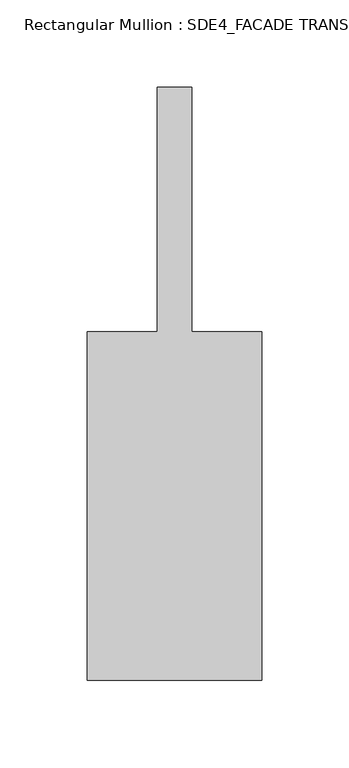
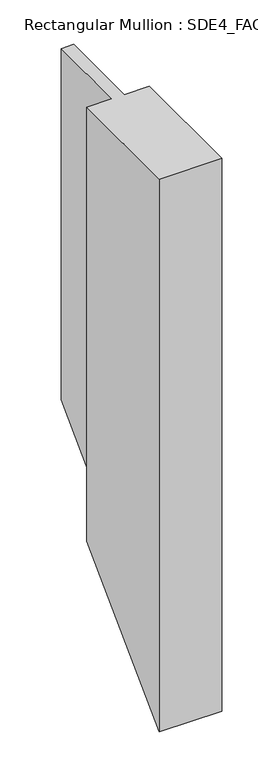
"""IFC4 building model written with IfcOpenShell, lengths in millimetres: member geometry, Rectangular Mullion : SDE4_FACADE TRANSOM TYPE 1."""

import ifcopenshell
import ifcopenshell.guid

model = None  # the IFC model being written
_history = None  # IfcOwnerHistory: only IFC2X3 demands one
_inside = {}  # id of a spatial element -> (the spatial element, [elements in it])
_under = {}  # id of a project, library or spatial element -> (it, [spatial elements below it])
_declared = {}  # id of a project -> (the project, [libraries it declares])
_typed = {}  # id of a type object -> (the type object, [elements of that type])
_made_of = {}  # id of a material, layer set ... -> (it, [elements and type objects made of it])


def new_model(schema):
    """Start an empty IFC model of exactly this schema.

    Asked for "IFC4X3", IfcOpenShell would pick the latest addendum, in which some entities
    have other attributes; the version numbers below select the first issue.
    IFC2X3 requires an IfcOwnerHistory on every rooted entity: one is made here for all.
    """
    global model, _history
    if schema == "IFC4X3":
        model = ifcopenshell.file(schema_version=(4, 3, 0, 0))
    else:
        model = ifcopenshell.file(schema=schema)
    _inside.clear()
    _under.clear()
    _declared.clear()
    _typed.clear()
    _made_of.clear()
    _history = None
    if model.schema == "IFC2X3":
        org = make("IfcOrganization", Name="unknown")
        user = make(
            "IfcPersonAndOrganization",
            ThePerson=make("IfcPerson", FamilyName="unknown"),
            TheOrganization=org,
        )
        app = make(
            "IfcApplication",
            ApplicationDeveloper=org,
            Version="unknown",
            ApplicationFullName="unknown",
            ApplicationIdentifier="unknown",
        )
        _history = make(
            "IfcOwnerHistory",
            OwningUser=user,
            OwningApplication=app,
            ChangeAction="ADDED",
            CreationDate=0,
        )
    return model


def make(cls, **values):
    """One entity of the class cls with the attributes given. An attribute that is None is left unset."""
    return model.create_entity(
        cls, **{name: value for name, value in values.items() if value is not None}
    )


def rooted(cls, **values):
    """An entity with a GlobalId (a new one), such as an element, a storey or a relation."""
    return make(cls, GlobalId=ifcopenshell.guid.new(), OwnerHistory=_history, **values)


def si_unit(unit_type, name, prefix=None):
    """IfcSIUnit, for example si_unit("LENGTHUNIT", "METRE", prefix="MILLI")."""
    return make("IfcSIUnit", UnitType=unit_type, Prefix=prefix, Name=name)


def assignment(units):
    """IfcUnitAssignment: the units of a project."""
    return None if units is None else make("IfcUnitAssignment", Units=units)


def point(xyz):
    """IfcCartesianPoint."""
    return None if xyz is None else make("IfcCartesianPoint", Coordinates=xyz)


def direction(xyz):
    """IfcDirection."""
    return None if xyz is None else make("IfcDirection", DirectionRatios=xyz)


def frame(location, z_axis=None, x_axis=None):
    """IfcAxis2Placement3D, a coordinate frame: its origin and axes. An axis left out is left unset."""
    return make(
        "IfcAxis2Placement3D",
        Location=point(location),
        Axis=direction(z_axis),
        RefDirection=direction(x_axis),
    )


def origin():
    """The frame at (0, 0, 0) with its axes left unset."""
    return frame((0.0, 0.0, 0.0))


def place(relative_to, where):
    """IfcLocalPlacement: puts the frame where relative to a parent placement (None: the world)."""
    return make(
        "IfcLocalPlacement", PlacementRelTo=relative_to, RelativePlacement=where
    )


def context(
    kind, dimensions, precision=None, world=None, true_north=None, identifier=None
):
    """IfcGeometricRepresentationContext, for example the 3D "Model" context."""
    return make(
        "IfcGeometricRepresentationContext",
        ContextIdentifier=identifier,
        ContextType=kind,
        CoordinateSpaceDimension=dimensions,
        Precision=precision,
        WorldCoordinateSystem=world,
        TrueNorth=true_north,
    )


def project(units=None, contexts=None):
    """IfcProject with its units and contexts."""
    return rooted(
        "IfcProject",
        Name="project",
        RepresentationContexts=contexts,
        UnitsInContext=assignment(units),
    )


def spatial(cls, under=None, at=None, **own):
    """A site, building, storey or space (cls), placed at a placement, below another one or the project."""
    s = rooted(cls, ObjectPlacement=at, **own)
    if under is not None:
        _under.setdefault(under.id(), (under, []))[1].append(s)
    return s


def faces_of(points, faces, orient=None, outer=None):
    """IfcFace entities. A face is a list of loops; a loop is a list of indices into points, from 0.

    orient and outer hold one flag for each loop. By default every Orientation is true, the
    first loop of a face is its IfcFaceOuterBound and the others are IfcFaceBound.
    """
    made = []
    for i, loops in enumerate(faces):
        bounds = []
        for j, loop in enumerate(loops):
            is_outer = j == 0 if outer is None else outer[i][j]
            bounds.append(
                make(
                    "IfcFaceOuterBound" if is_outer else "IfcFaceBound",
                    Bound=make("IfcPolyLoop", Polygon=[points[k] for k in loop]),
                    Orientation=True if orient is None else orient[i][j],
                )
            )
        made.append(make("IfcFace", Bounds=bounds))
    return made


def faceted_brep(points, faces, orient=None, outer=None, voids=None):
    """IfcFacetedBrep: a solid bounded by flat faces; with voids (closed shells), ...WithVoids."""
    shared = [point(p) for p in points]
    hull = make("IfcClosedShell", CfsFaces=faces_of(shared, faces, orient, outer))
    if voids is None:
        return make("IfcFacetedBrep", Outer=hull)
    return make(
        "IfcFacetedBrepWithVoids",
        Outer=hull,
        Voids=[
            make(cls, CfsFaces=faces_of(shared, fs, o, b)) for cls, fs, o, b in voids
        ],
    )


def shape(context_of_items, identifier, shape_type, items):
    """IfcShapeRepresentation: the items that make up one representation, for example the "Body"."""
    return make(
        "IfcShapeRepresentation",
        ContextOfItems=context_of_items,
        RepresentationIdentifier=identifier,
        RepresentationType=shape_type,
        Items=items,
    )


def source(mapping_origin, context_of_items, identifier, shape_type, items):
    """IfcRepresentationMap: a shape defined once, which mapped items show again and again."""
    return make(
        "IfcRepresentationMap",
        MappingOrigin=mapping_origin,
        MappedRepresentation=shape(context_of_items, identifier, shape_type, items),
    )


def transform(
    local_origin,
    x_axis=None,
    y_axis=None,
    z_axis=None,
    scale=None,
    scale2=None,
    scale3=None,
    uniform=True,
):
    """IfcCartesianTransformationOperator3D, or its non-uniform kind. x_axis, y_axis, z_axis: its Axis1, 2, 3."""
    if uniform:
        return make(
            "IfcCartesianTransformationOperator3D",
            Axis1=direction(x_axis),
            Axis2=direction(y_axis),
            LocalOrigin=point(local_origin),
            Scale=scale,
            Axis3=direction(z_axis),
        )
    return make(
        "IfcCartesianTransformationOperator3DnonUniform",
        Axis1=direction(x_axis),
        Axis2=direction(y_axis),
        LocalOrigin=point(local_origin),
        Scale=scale,
        Axis3=direction(z_axis),
        Scale2=scale2,
        Scale3=scale3,
    )


def mapped(mapping_source, mapping_target):
    """IfcMappedItem: shows the shape of a source again, moved by a transform."""
    return make(
        "IfcMappedItem", MappingSource=mapping_source, MappingTarget=mapping_target
    )


def made_of(thing, what):
    """Note that an element or type object is made of a material, layer set ...; save() writes the relation."""
    if what is not None:
        _made_of.setdefault(what.id(), (what, []))[1].append(thing)
    return thing


def element(
    cls,
    number,
    at=None,
    inside=None,
    cuts=None,
    type_object=None,
    material=None,
    context=None,
    identifier="Body",
    shape_type=None,
    held_by="IfcProductDefinitionShape",
    body=None,
    shapes=None,
    **own,
):
    """One element of the class cls, such as IfcWall. Its Tag is "e" and its number.

    at: its placement. inside: the storey or other place that contains it. cuts: it is an
    opening in that element (IfcRelVoidsElement). A single representation is given by context,
    identifier, shape_type and body (its items); several are given by shapes. held_by: the class
    of the entity that holds the representations. save() writes the other relations.
    """
    e = rooted(cls, Tag="e%d" % number, ObjectPlacement=at, **own)
    if body is not None:
        shapes = [shape(context, identifier, shape_type, body)]
    if shapes is not None:
        e.Representation = make(held_by, Representations=shapes)
    if inside is not None:
        _inside.setdefault(inside.id(), (inside, []))[1].append(e)
    if cuts is not None:
        rooted(
            "IfcRelVoidsElement", RelatingBuildingElement=cuts, RelatedOpeningElement=e
        )
    if type_object is not None:
        _typed.setdefault(type_object.id(), (type_object, []))[1].append(e)
    return made_of(e, material)


def aggregate(whole, parts):
    """IfcRelAggregates: a whole, such as a stair, and the parts it consists of."""
    return rooted("IfcRelAggregates", RelatingObject=whole, RelatedObjects=parts)


def save(model, path):
    """Write the relations noted so far, then the file.

    IfcRelAggregates (storeys below a building ...), IfcRelContainedInSpatialStructure (elements
    in a storey), IfcRelDefinesByType, IfcRelAssociatesMaterial and IfcRelDeclares: one each for
    every whole, place, type object, material and project.
    """
    for whole, parts in _under.values():
        aggregate(whole, parts)
    for where, things in _inside.values():
        rooted(
            "IfcRelContainedInSpatialStructure",
            RelatedElements=things,
            RelatingStructure=where,
        )
    for kind, things in _typed.values():
        rooted("IfcRelDefinesByType", RelatedObjects=things, RelatingType=kind)
    for what, things in _made_of.values():
        rooted("IfcRelAssociatesMaterial", RelatedObjects=things, RelatingMaterial=what)
    for by, libraries in _declared.values():
        rooted("IfcRelDeclares", RelatingContext=by, RelatedDefinitions=libraries)
    model.write(path)


def rectangular_mullion_sde4_facade_transom_type_1_d566cc6e(model_context):
    return source(origin(), model_context, "Body", "Brep", [
        faceted_brep([(50.0, -132.5, 0.0), (50.0, 67.5, 0.0), (10.0, 67.5, 0.0), (10.0, 207.5, 0.0), (-10.0, 207.5, 0.0), (-10.0, 67.5, 0.0), (-50.0, 67.5, 0.0), (-50.0, -132.5, 0.0), (50.0, -132.5, -932.9646548), (50.0, 67.5, -732.9646548), (10.0, 67.5, -732.9646548), (10.0, 207.5, -592.9646548), (-10.0, 207.5, -592.9646548), (-10.0, 67.5, -732.9646548), (-50.0, 67.5, -732.9646548), (-50.0, -132.5, -932.9646548)], [[[0, 1, 2, 3, 4, 5, 6, 7]], [[1, 0, 8, 9]], [[2, 1, 9, 10]], [[3, 2, 10, 11]], [[4, 3, 11, 12]], [[5, 4, 12, 13]], [[6, 5, 13, 14]], [[7, 6, 14, 15]], [[0, 7, 15, 8]], [[8, 15, 14, 13, 12, 11, 10, 9]]]),
    ])


if __name__ == "__main__":
    model = new_model("IFC4")
    model_context = context("Model", 3, world=origin())
    ifc_project = project(units=[si_unit("LENGTHUNIT", "METRE", prefix="MILLI")], contexts=[model_context])
    site = spatial("IfcSite", under=ifc_project)
    building = spatial("IfcBuilding", under=site)
    placement = place(None, origin())
    rectangular_mullion_sde4_facade_transom_type_1_shape = rectangular_mullion_sde4_facade_transom_type_1_d566cc6e(model_context)
    element("IfcMember", 1, ObjectType="Rectangular Mullion : SDE4_FACADE TRANSOM TYPE 1", at=placement, inside=building, context=model_context, shape_type="MappedRepresentation", body=[
        mapped(rectangular_mullion_sde4_facade_transom_type_1_shape, transform((0.0, 0.0, 0.0), x_axis=(1.0, 0.0, 0.0), y_axis=(0.0, 1.0, 0.0), z_axis=(0.0, 0.0, 1.0))),
    ])
    save(model, "model.ifc")

# Revit data of these elements
# Type "Rectangular Mullion : SDE4_FACADE TRANSOM TYPE 1"
#   built-in parameter 1007322 = 1.11549 (stored number, unit not read)
#   built-in parameter 1007321 = 0.164042 (stored number, unit not read)
#   built-in parameter 1007320 = 0.164042 (stored number, unit not read)
